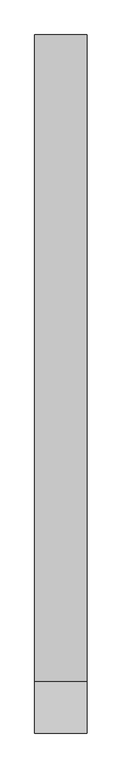
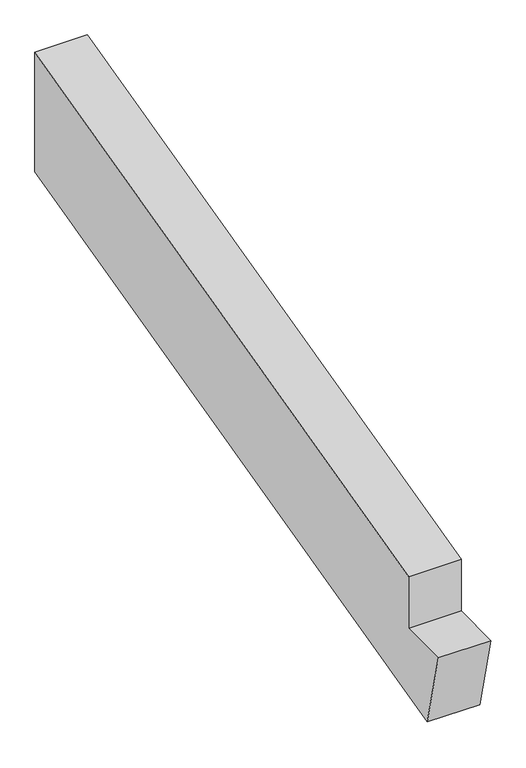
"""IFC4 building model written with IfcOpenShell, lengths in millimetres: proxy geometry, Framing7:Framing025:286338 : Framing7:Framing025:286338."""

from ifc_helpers import new_model, si_unit, frame, origin, place, context, project, spatial, polyline, outline, extrude, source, transform, mapped, element, save


def generic_models_d0207d18(model_context):
    return source(origin(), model_context, "Body", "SweptSolid", [
        extrude(outline(polyline([(-5040.1231329, 42411.3663805), (-5096.6420486, 42642.0307603), (-4946.0750638, 42642.0307603), (-4946.0750638, 42800.8143799), (-3066.3240751, 43270.717426), (-3066.3240751, 42903.8818003), (-5040.1231329, 42411.3663805)])), frame((17311.909108, 0.0, 0.0), z_axis=(1.0, 0.0, 0.0), x_axis=(0.0, 1.0, 0.0)), (0.0, 0.0, 1.0), 152.4),
    ])


if __name__ == "__main__":
    model = new_model("IFC4")
    model_context = context("Model", 3, world=origin())
    ifc_project = project(units=[si_unit("LENGTHUNIT", "METRE", prefix="MILLI")], contexts=[model_context])
    site = spatial("IfcSite", under=ifc_project)
    building = spatial("IfcBuilding", under=site)
    placement = place(None, origin())
    generic_models_shape = generic_models_d0207d18(model_context)
    element("IfcBuildingElementProxy", 1, Name="Framing7:Framing025:286338 : Framing7:Framing025:286338", ObjectType="Framing7:Framing025:286338 : Framing7:Framing025:286338", at=placement, inside=building, context=model_context, shape_type="MappedRepresentation", body=[
        mapped(generic_models_shape, transform((0.0, 0.0, 0.0), x_axis=(1.0, 0.0, 0.0), y_axis=(0.0, 1.0, 0.0), z_axis=(0.0, 0.0, 1.0))),
    ])
    save(model, "model.ifc")

# Revit data of these elements
# Type "Framing7:Framing025:286338 : Framing7:Framing025:286338"
#   NameOverride = "Framing7:Framing025:286338"
#   ObjectTypeOverride = "Framing7:Framing025"
#   Reference = "Framing025"
#   Category = "Generic Models"
#   Tag = "286338"
# Element 1 (IfcBuildingElementProxy, "Framing7:Framing025:286338 : Framing7:Framing025:286338")
#   Materials on its faces: "WOOD FRAMING (SEE STRUCT DWGS)"
# Materials
#   "WOOD FRAMING (SEE STRUCT DWGS)": class "Unassigned", colour RGB 224 188 168, transparency 0, Cost = 0
